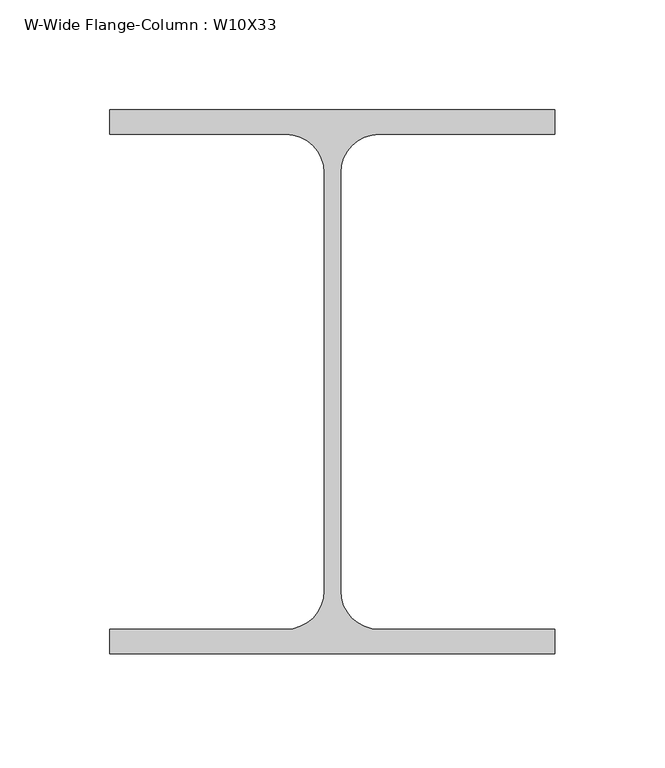
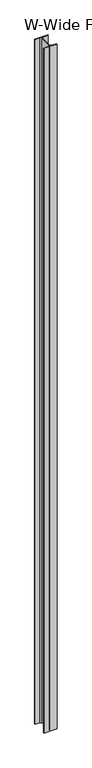
"""IFC4 building model written with IfcOpenShell, lengths in millimetres: column geometry, W-Wide Flange-Column : W10X33."""

from ifc_helpers import new_model, si_unit, point, frame, frame_2d, origin, place, context, project, spatial, polyline, circle_curve, trimmed, segment, composite_curve, outline, extrude, source, transform, mapped, element, save


def w_wide_flange_column_w10x33_a2e74f78(model_context):
    return source(origin(), model_context, "Body", "SweptSolid", [
        extrude(outline(composite_curve([segment(polyline([(101.092, 123.571), (101.092, 112.522), (21.209, 112.522)]), True, "CONTINUOUS"), segment(trimmed(circle_curve(frame_2d((21.209, 94.996)), 17.526), [point((21.209, 112.522))], [point((3.683, 94.996))], True, "CARTESIAN"), True, "CONTINUOUS"), segment(polyline([(3.683, 94.996), (3.683, -94.996)]), True, "CONTINUOUS"), segment(trimmed(circle_curve(frame_2d((21.209, -94.996)), 17.526), [point((3.683, -94.996))], [point((21.209, -112.522))], True, "CARTESIAN"), True, "CONTINUOUS"), segment(polyline([(21.209, -112.522), (101.092, -112.522), (101.092, -123.571), (-101.092, -123.571), (-101.092, -112.522), (-21.209, -112.522)]), True, "CONTINUOUS"), segment(trimmed(circle_curve(frame_2d((-21.209, -94.996)), 17.526), [point((-21.209, -112.522))], [point((-3.683, -94.996))], True, "CARTESIAN"), True, "CONTINUOUS"), segment(polyline([(-3.683, -94.996), (-3.683, 94.996)]), True, "CONTINUOUS"), segment(trimmed(circle_curve(frame_2d((-21.209, 94.996)), 17.526), [point((-3.683, 94.996))], [point((-21.209, 112.522))], True, "CARTESIAN"), True, "CONTINUOUS"), segment(polyline([(-21.209, 112.522), (-101.092, 112.522), (-101.092, 123.571), (101.092, 123.571)]), True, "CONTINUOUS")], self_intersect=False)), frame((0.0, 0.0, 16408.4), z_axis=(0.0, 0.0, 1.0), x_axis=(1.0, 0.0, 0.0)), (0.0, 0.0, 1.0), 11176.0),
    ])


if __name__ == "__main__":
    model = new_model("IFC4")
    model_context = context("Model", 3, world=origin())
    ifc_project = project(units=[si_unit("LENGTHUNIT", "METRE", prefix="MILLI")], contexts=[model_context])
    site = spatial("IfcSite", under=ifc_project)
    building = spatial("IfcBuilding", under=site)
    placement = place(None, origin())
    w_wide_flange_column_w10x33_shape = w_wide_flange_column_w10x33_a2e74f78(model_context)
    element("IfcColumn", 1, ObjectType="W-Wide Flange-Column : W10X33", at=placement, inside=building, context=model_context, shape_type="MappedRepresentation", body=[
        mapped(w_wide_flange_column_w10x33_shape, transform((0.0, 0.0, 0.0), x_axis=(1.0, 0.0, 0.0), y_axis=(0.0, 1.0, 0.0), z_axis=(0.0, 0.0, 1.0))),
    ])
    save(model, "model.ifc")

# Revit data of these elements
# Type "W-Wide Flange-Column : W10X33"
#   Assembly Code = "B10"
#   W = 33
#   bf = 0' - 7.96"
#   d = 0' - 9.73"
#   k = 0' - 1 1/8"
#   kr = 0' - 0.69"
#   tf = 0' - 0.435"
#   tw = 0' - 0.29"
#   A = 0.0674306 SF
#   Structural Material [instance default] = Steel ASTM A992
# Element 1 (IfcColumn, "W-Wide Flange-Column : W10X33")
#   Materials on its faces: "Steel ASTM A992"
# Materials
#   "Steel ASTM A992": class "Metal", colour RGB 199 199 199, transparency 0, Description = "Structural steel 50ksi", Cost = 0
